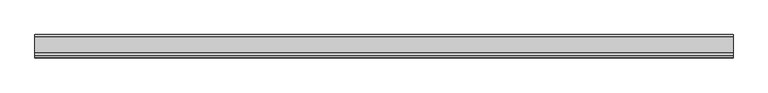
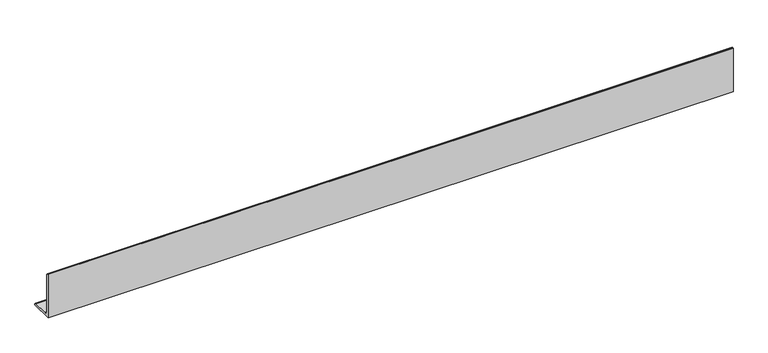
"""IFC4 building model written with IfcOpenShell, lengths in millimetres: beam geometry, NLRS_28_SF_LIB_stalen ligger hoekprofiel ongelijkzijdig-AV-MMBS-SRP_gen_rsf : stalen ligger ongelijzijdig hoekprofiel LUEQ_gen__200x100x10."""

import ifcopenshell
import ifcopenshell.guid

model = None  # the IFC model being written
_history = None  # IfcOwnerHistory: only IFC2X3 demands one
_inside = {}  # id of a spatial element -> (the spatial element, [elements in it])
_under = {}  # id of a project, library or spatial element -> (it, [spatial elements below it])
_declared = {}  # id of a project -> (the project, [libraries it declares])
_typed = {}  # id of a type object -> (the type object, [elements of that type])
_made_of = {}  # id of a material, layer set ... -> (it, [elements and type objects made of it])


def new_model(schema):
    """Start an empty IFC model of exactly this schema.

    Asked for "IFC4X3", IfcOpenShell would pick the latest addendum, in which some entities
    have other attributes; the version numbers below select the first issue.
    IFC2X3 requires an IfcOwnerHistory on every rooted entity: one is made here for all.
    """
    global model, _history
    if schema == "IFC4X3":
        model = ifcopenshell.file(schema_version=(4, 3, 0, 0))
    else:
        model = ifcopenshell.file(schema=schema)
    _inside.clear()
    _under.clear()
    _declared.clear()
    _typed.clear()
    _made_of.clear()
    _history = None
    if model.schema == "IFC2X3":
        org = make("IfcOrganization", Name="unknown")
        user = make(
            "IfcPersonAndOrganization",
            ThePerson=make("IfcPerson", FamilyName="unknown"),
            TheOrganization=org,
        )
        app = make(
            "IfcApplication",
            ApplicationDeveloper=org,
            Version="unknown",
            ApplicationFullName="unknown",
            ApplicationIdentifier="unknown",
        )
        _history = make(
            "IfcOwnerHistory",
            OwningUser=user,
            OwningApplication=app,
            ChangeAction="ADDED",
            CreationDate=0,
        )
    return model


def make(cls, **values):
    """One entity of the class cls with the attributes given. An attribute that is None is left unset."""
    return model.create_entity(
        cls, **{name: value for name, value in values.items() if value is not None}
    )


def rooted(cls, **values):
    """An entity with a GlobalId (a new one), such as an element, a storey or a relation."""
    return make(cls, GlobalId=ifcopenshell.guid.new(), OwnerHistory=_history, **values)


def si_unit(unit_type, name, prefix=None):
    """IfcSIUnit, for example si_unit("LENGTHUNIT", "METRE", prefix="MILLI")."""
    return make("IfcSIUnit", UnitType=unit_type, Prefix=prefix, Name=name)


def assignment(units):
    """IfcUnitAssignment: the units of a project."""
    return None if units is None else make("IfcUnitAssignment", Units=units)


def point(xyz):
    """IfcCartesianPoint."""
    return None if xyz is None else make("IfcCartesianPoint", Coordinates=xyz)


def direction(xyz):
    """IfcDirection."""
    return None if xyz is None else make("IfcDirection", DirectionRatios=xyz)


def frame(location, z_axis=None, x_axis=None):
    """IfcAxis2Placement3D, a coordinate frame: its origin and axes. An axis left out is left unset."""
    return make(
        "IfcAxis2Placement3D",
        Location=point(location),
        Axis=direction(z_axis),
        RefDirection=direction(x_axis),
    )


def frame_2d(location, x_axis=None):
    """IfcAxis2Placement2D, a coordinate frame in the plane: its origin and x axis."""
    return make(
        "IfcAxis2Placement2D", Location=point(location), RefDirection=direction(x_axis)
    )


def origin():
    """The frame at (0, 0, 0) with its axes left unset."""
    return frame((0.0, 0.0, 0.0))


def place(relative_to, where):
    """IfcLocalPlacement: puts the frame where relative to a parent placement (None: the world)."""
    return make(
        "IfcLocalPlacement", PlacementRelTo=relative_to, RelativePlacement=where
    )


def context(
    kind, dimensions, precision=None, world=None, true_north=None, identifier=None
):
    """IfcGeometricRepresentationContext, for example the 3D "Model" context."""
    return make(
        "IfcGeometricRepresentationContext",
        ContextIdentifier=identifier,
        ContextType=kind,
        CoordinateSpaceDimension=dimensions,
        Precision=precision,
        WorldCoordinateSystem=world,
        TrueNorth=true_north,
    )


def project(units=None, contexts=None):
    """IfcProject with its units and contexts."""
    return rooted(
        "IfcProject",
        Name="project",
        RepresentationContexts=contexts,
        UnitsInContext=assignment(units),
    )


def spatial(cls, under=None, at=None, **own):
    """A site, building, storey or space (cls), placed at a placement, below another one or the project."""
    s = rooted(cls, ObjectPlacement=at, **own)
    if under is not None:
        _under.setdefault(under.id(), (under, []))[1].append(s)
    return s


def polyline(points):
    """IfcPolyline through the points."""
    return make("IfcPolyline", Points=[point(p) for p in points])


def circle_curve(where, radius):
    """IfcCircle in the frame where."""
    return make("IfcCircle", Position=where, Radius=radius)


def trimmed(basis, trim1, trim2, sense, master):
    """IfcTrimmedCurve: the piece of a basis curve between two trims."""
    return make(
        "IfcTrimmedCurve",
        BasisCurve=basis,
        Trim1=trim1,
        Trim2=trim2,
        SenseAgreement=sense,
        MasterRepresentation=master,
    )


def segment(curve, same_sense, transition):
    """IfcCompositeCurveSegment."""
    return make(
        "IfcCompositeCurveSegment",
        Transition=transition,
        SameSense=same_sense,
        ParentCurve=curve,
    )


def composite_curve(segments, self_intersect=None):
    """IfcCompositeCurve: segments joined end to end."""
    return make("IfcCompositeCurve", Segments=segments, SelfIntersect=self_intersect)


def outline(outer, holes=None, kind="AREA"):
    """IfcArbitraryClosedProfileDef: a profile drawn as a closed curve; with holes, ...WithVoids."""
    if holes is None:
        return make("IfcArbitraryClosedProfileDef", ProfileType=kind, OuterCurve=outer)
    return make(
        "IfcArbitraryProfileDefWithVoids",
        ProfileType=kind,
        OuterCurve=outer,
        InnerCurves=holes,
    )


def extrude(swept, where, along, depth):
    """IfcExtrudedAreaSolid: the profile swept, set in the frame where, extruded along a direction by depth."""
    return make(
        "IfcExtrudedAreaSolid",
        SweptArea=swept,
        Position=where,
        ExtrudedDirection=direction(along),
        Depth=depth,
    )


def shape(context_of_items, identifier, shape_type, items):
    """IfcShapeRepresentation: the items that make up one representation, for example the "Body"."""
    return make(
        "IfcShapeRepresentation",
        ContextOfItems=context_of_items,
        RepresentationIdentifier=identifier,
        RepresentationType=shape_type,
        Items=items,
    )


def source(mapping_origin, context_of_items, identifier, shape_type, items):
    """IfcRepresentationMap: a shape defined once, which mapped items show again and again."""
    return make(
        "IfcRepresentationMap",
        MappingOrigin=mapping_origin,
        MappedRepresentation=shape(context_of_items, identifier, shape_type, items),
    )


def transform(
    local_origin,
    x_axis=None,
    y_axis=None,
    z_axis=None,
    scale=None,
    scale2=None,
    scale3=None,
    uniform=True,
):
    """IfcCartesianTransformationOperator3D, or its non-uniform kind. x_axis, y_axis, z_axis: its Axis1, 2, 3."""
    if uniform:
        return make(
            "IfcCartesianTransformationOperator3D",
            Axis1=direction(x_axis),
            Axis2=direction(y_axis),
            LocalOrigin=point(local_origin),
            Scale=scale,
            Axis3=direction(z_axis),
        )
    return make(
        "IfcCartesianTransformationOperator3DnonUniform",
        Axis1=direction(x_axis),
        Axis2=direction(y_axis),
        LocalOrigin=point(local_origin),
        Scale=scale,
        Axis3=direction(z_axis),
        Scale2=scale2,
        Scale3=scale3,
    )


def mapped(mapping_source, mapping_target):
    """IfcMappedItem: shows the shape of a source again, moved by a transform."""
    return make(
        "IfcMappedItem", MappingSource=mapping_source, MappingTarget=mapping_target
    )


def made_of(thing, what):
    """Note that an element or type object is made of a material, layer set ...; save() writes the relation."""
    if what is not None:
        _made_of.setdefault(what.id(), (what, []))[1].append(thing)
    return thing


def element(
    cls,
    number,
    at=None,
    inside=None,
    cuts=None,
    type_object=None,
    material=None,
    context=None,
    identifier="Body",
    shape_type=None,
    held_by="IfcProductDefinitionShape",
    body=None,
    shapes=None,
    **own,
):
    """One element of the class cls, such as IfcWall. Its Tag is "e" and its number.

    at: its placement. inside: the storey or other place that contains it. cuts: it is an
    opening in that element (IfcRelVoidsElement). A single representation is given by context,
    identifier, shape_type and body (its items); several are given by shapes. held_by: the class
    of the entity that holds the representations. save() writes the other relations.
    """
    e = rooted(cls, Tag="e%d" % number, ObjectPlacement=at, **own)
    if body is not None:
        shapes = [shape(context, identifier, shape_type, body)]
    if shapes is not None:
        e.Representation = make(held_by, Representations=shapes)
    if inside is not None:
        _inside.setdefault(inside.id(), (inside, []))[1].append(e)
    if cuts is not None:
        rooted(
            "IfcRelVoidsElement", RelatingBuildingElement=cuts, RelatedOpeningElement=e
        )
    if type_object is not None:
        _typed.setdefault(type_object.id(), (type_object, []))[1].append(e)
    return made_of(e, material)


def aggregate(whole, parts):
    """IfcRelAggregates: a whole, such as a stair, and the parts it consists of."""
    return rooted("IfcRelAggregates", RelatingObject=whole, RelatedObjects=parts)


def save(model, path):
    """Write the relations noted so far, then the file.

    IfcRelAggregates (storeys below a building ...), IfcRelContainedInSpatialStructure (elements
    in a storey), IfcRelDefinesByType, IfcRelAssociatesMaterial and IfcRelDeclares: one each for
    every whole, place, type object, material and project.
    """
    for whole, parts in _under.values():
        aggregate(whole, parts)
    for where, things in _inside.values():
        rooted(
            "IfcRelContainedInSpatialStructure",
            RelatedElements=things,
            RelatingStructure=where,
        )
    for kind, things in _typed.values():
        rooted("IfcRelDefinesByType", RelatedObjects=things, RelatingType=kind)
    for what, things in _made_of.values():
        rooted("IfcRelAssociatesMaterial", RelatedObjects=things, RelatingMaterial=what)
    for by, libraries in _declared.values():
        rooted("IfcRelDeclares", RelatingContext=by, RelatedDefinitions=libraries)
    model.write(path)


def beam_d9217694(model_context):
    return source(origin(), model_context, "Body", "SweptSolid", [
        extrude(outline(composite_curve([segment(polyline([(-20.13, -69.3), (-20.13, 130.7), (-17.63, 130.7)]), True, "CONTINUOUS"), segment(trimmed(circle_curve(frame_2d((-17.63, 123.2)), 7.5), [point((-17.63, 130.7))], [point((-10.13, 123.2))], False, "CARTESIAN"), True, "CONTINUOUS"), segment(polyline([(-10.13, 123.2), (-10.13, -44.3)]), True, "CONTINUOUS"), segment(trimmed(circle_curve(frame_2d((4.87, -44.3)), 15.0), [point((-10.13, -44.3))], [point((4.87, -59.3))], True, "CARTESIAN"), True, "CONTINUOUS"), segment(polyline([(4.87, -59.3), (72.37, -59.3)]), True, "CONTINUOUS"), segment(trimmed(circle_curve(frame_2d((72.37, -66.8)), 7.5), [point((72.37, -59.3))], [point((79.87, -66.8))], False, "CARTESIAN"), True, "CONTINUOUS"), segment(polyline([(79.87, -66.8), (79.87, -69.3), (-20.13, -69.3)]), True, "CONTINUOUS")], self_intersect=False)), frame((-1482.2999994, 0.0, 0.0), z_axis=(1.0, 0.0, 0.0), x_axis=(0.0, 1.0, 0.0)), (0.0, 0.0, 1.0), 2977.2999994),
    ])


if __name__ == "__main__":
    model = new_model("IFC4")
    model_context = context("Model", 3, world=origin())
    ifc_project = project(units=[si_unit("LENGTHUNIT", "METRE", prefix="MILLI")], contexts=[model_context])
    site = spatial("IfcSite", under=ifc_project)
    building = spatial("IfcBuilding", under=site)
    placement = place(None, origin())
    beam_shape = beam_d9217694(model_context)
    element("IfcBeam", 1, ObjectType="NLRS_28_SF_LIB_stalen ligger hoekprofiel ongelijkzijdig-AV-MMBS-SRP_gen_rsf : stalen ligger ongelijzijdig hoekprofiel LUEQ_gen__200x100x10", at=placement, inside=building, context=model_context, shape_type="MappedRepresentation", body=[
        mapped(beam_shape, transform((0.0, 0.0, 0.0), x_axis=(1.0, 0.0, 0.0), y_axis=(0.0, 1.0, 0.0), z_axis=(0.0, 0.0, 1.0))),
    ])
    save(model, "model.ifc")

# Revit data of these elements
# Type "NLRS_28_SF_LIB_stalen ligger hoekprofiel ongelijkzijdig-AV-MMBS-SRP_gen_rsf : stalen ligger ongelijzijdig hoekprofiel LUEQ_gen__200x100x10"
#   Export Type to IFC As = "IfcBeamType"
#   Type IfcGUID = "0dxhH9VHH5jh7XQ0uLfXuR"
#   Type Comments = "L200x100x10"
#   Model = " "
#   Manufacturer = " "
#   Fire Rating = " "
#   Description = "stalen ligger L200x100x10"
#   Assembly Code = "28.11"
#   vz = 130.7 mm
#   vy = 79.87 mm
#   tw = 10 mm
#   tf = 10 mm
#   ri = 7.5 mm
#   ra = 15 mm
#   d = 200 mm
#   bf = 100 mm
#   NLRS_C_lengte [instance default] = 1524 mm
#   Length [instance default] = 1524 mm
#   Structural Material = NLRS_h2_staal_gen_rsf
#   Keynote = ""
# Element 1 (IfcBeam, "NLRS_28_SF_LIB_stalen ligger hoekprofiel ongelijkzijdig-AV-MMBS-SRP_gen_rsf : stalen ligger ongelijzijdig hoekprofiel LUEQ_gen__200x100x10")
#   NLRS_C_lengte = 2990 mm
#   Materials on its faces: "NLRS_h2_staal_gen_rsf"
# Materials
#   "NLRS_h2_staal_gen_rsf": class "H - Metaal", colour RGB 189 187 185, transparency 0, Keynote = "h2", Manufacturer = "Revit Standards Foundation", URL = "www.revitstandards.org", Description = "staal", Cost = 0
